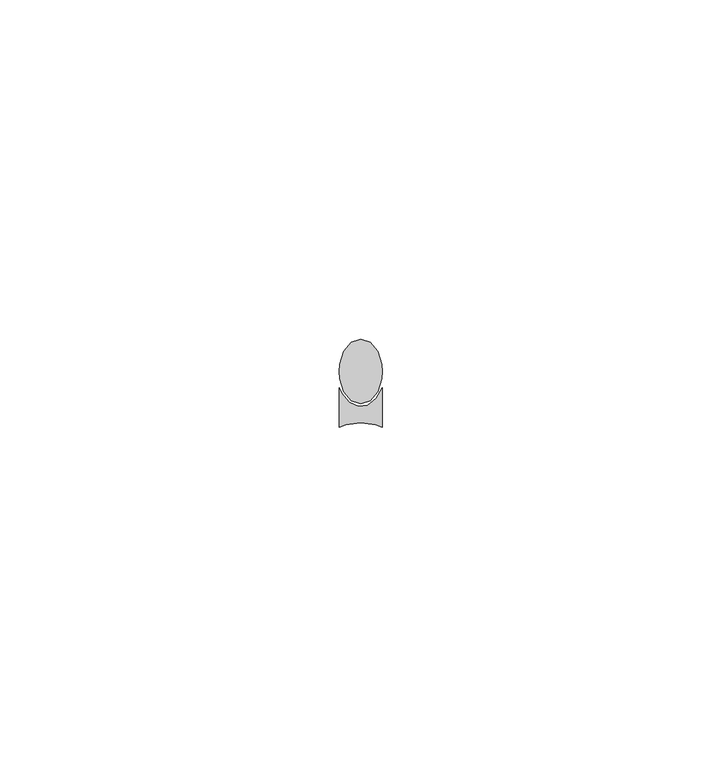
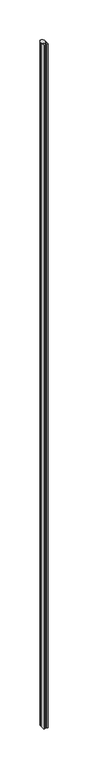
"""IFC4 building model written with IfcOpenShell, lengths in millimetres: proxy geometry, Generic Models 11:Generic Models 1:306267:Generic Models 1:306267 : Generic Models 11:Generic Models 1:306267:300405:Generic Models 1:306267:Generic Models 1:306267 : Generic Models 11:Generic Models 1:306267:300405 : Generic Models 11:Generic Models 1:306267:Generic Models 1:306267 : Generic Models 11:Generic Models 1:306267:300405:21 : Generic Models 11:Generic Models 1:306267:Generic Models 1:306267 : Generic Models 11:Generic Models 1:306267:300405:Generic Models 1:306267:Generic Models 1:306267 : Generic Models 11:Generic Models 1:306267:300405 : Generic Models 11:Generic Models 1:306267:Generic Models 1:306267 : Generic Models 11:Generic Models 1:306267:300405:300182."""

from ifc_helpers import new_model, si_unit, frame, origin, place, context, project, spatial, polyline, outline, extrude, source, transform, mapped, element, save


def generic_models_baf57337(model_context):
    return source(origin(), model_context, "Body", "SweptSolid", [
        extrude(outline(polyline([(593733.5341431, -579092.0005286), (593732.429409, -579090.6790346), (593731.8163278, -579088.7694203), (593731.7367239, -579087.7096644), (593731.8163278, -579086.6499084), (593732.429409, -579084.7402942), (593733.5341431, -579083.4188002), (593734.9117239, -579082.9471644), (593736.2893048, -579083.4188002), (593737.3940389, -579084.7402942), (593738.0071201, -579086.6499084), (593738.0867239, -579087.7096644), (593738.0071201, -579088.7694203), (593737.3940389, -579090.6790346), (593736.2893048, -579092.0005286), (593734.9117239, -579092.4721644), (593733.5341431, -579092.0005286)])), frame((0.0, 0.0, 5106.0759872), z_axis=(0.0, 0.0, 1.0), x_axis=(1.0, 0.0, 0.0)), (0.0, 0.0, 1.0), 1071.4379058),
        extrude(outline(polyline([(593737.1209607, -579095.5639755), (593734.9117239, -579095.2502894), (593732.7024872, -579095.5639755), (593731.7367239, -579095.9413841), (593731.7367239, -579090.073292), (593732.1230415, -579090.9335729), (593733.206527, -579092.2431481), (593734.5567747, -579092.8435016), (593735.962551, -579092.6407137), (593737.2039351, -579091.6665087), (593738.0867239, -579090.073292), (593738.0867239, -579095.9413841), (593737.1209607, -579095.5639755)])), frame((0.0, 0.0, 5106.0759872), z_axis=(0.0, 0.0, 1.0), x_axis=(1.0, 0.0, 0.0)), (0.0, 0.0, 1.0), 1071.4379058),
    ])


if __name__ == "__main__":
    model = new_model("IFC4")
    model_context = context("Model", 3, world=origin())
    ifc_project = project(units=[si_unit("LENGTHUNIT", "METRE", prefix="MILLI")], contexts=[model_context])
    site = spatial("IfcSite", under=ifc_project)
    building = spatial("IfcBuilding", under=site)
    placement = place(None, origin())
    generic_models_shape = generic_models_baf57337(model_context)
    element("IfcBuildingElementProxy", 1, Name="Generic Models 11:Generic Models 1:306267:Generic Models 1:306267 : Generic Models 11:Generic Models 1:306267:300405:Generic Models 1:306267:Generic Models 1:306267 : Generic Models 11:Generic Models 1:306267:300405 : Generic Models 11:Generic Models 1:306267:Generic Models 1:306267 : Generic Models 11:Generic Models 1:306267:300405:21 : Generic Models 11:Generic Models 1:306267:Generic Models 1:306267 : Generic Models 11:Generic Models 1:306267:300405:Generic Models 1:306267:Generic Models 1:306267 : Generic Models 11:Generic Models 1:306267:300405 : Generic Models 11:Generic Models 1:306267:Generic Models 1:306267 : Generic Models 11:Generic Models 1:306267:300405:300182", ObjectType="Generic Models 11:Generic Models 1:306267:Generic Models 1:306267 : Generic Models 11:Generic Models 1:306267:300405:Generic Models 1:306267:Generic Models 1:306267 : Generic Models 11:Generic Models 1:306267:300405 : Generic Models 11:Generic Models 1:306267:Generic Models 1:306267 : Generic Models 11:Generic Models 1:306267:300405:21 : Generic Models 11:Generic Models 1:306267:Generic Models 1:306267 : Generic Models 11:Generic Models 1:306267:300405:Generic Models 1:306267:Generic Models 1:306267 : Generic Models 11:Generic Models 1:306267:300405 : Generic Models 11:Generic Models 1:306267:Generic Models 1:306267 : Generic Models 11:Generic Models 1:306267:300405:300182", at=placement, inside=building, context=model_context, shape_type="MappedRepresentation", body=[
        mapped(generic_models_shape, transform((0.0, 0.0, 0.0), x_axis=(1.0, 0.0, 0.0), y_axis=(0.0, 1.0, 0.0), z_axis=(0.0, 0.0, 1.0))),
    ])
    save(model, "model.ifc")

# Revit data of these elements
# Type "Generic Models 11:Generic Models 1:306267:Generic Models 1:306267 : Generic Models 11:Generic Models 1:306267:300405:Generic Models 1:306267:Generic Models 1:306267 : Generic Models 11:Generic Models 1:306267:300405 : Generic Models 11:Generic Models 1:306267:Generic Models 1:306267 : Generic Models 11:Generic Models 1:306267:300405:21 : Generic Models 11:Generic Models 1:306267:Generic Models 1:306267 : Generic Models 11:Generic Models 1:306267:300405:Generic Models 1:306267:Generic Models 1:306267 : Generic Models 11:Generic Models 1:306267:300405 : Generic Models 11:Generic Models 1:306267:Generic Models 1:306267 : Generic Models 11:Generic Models 1:306267:300405:300182"
#   NameOverride = "Generic Models 11:Generic Models 1:306267:Generic Models 1:306267 : Generic Models 11:Generic Models 1:306267:300405:Generic Models 1:306267:Generic Models 1:306267 : Generic Models 11:Generic Models 1:306267:300405 : Generic Models 11:Generic Models 1:306267:Generic Models 1:306267 : Generic Models 11:Generic Models 1:306267:300405:300182"
#   ObjectTypeOverride = "Generic Models 1:306267:Generic Models 1:306267 : Generic Models 11:Generic Models 1:306267:300405 : Generic Models 11:Generic Models 1:306267:Generic Models 1:306267 : Generic Models 11:Generic Models 1:306267:300405"
#   Reference = "Generic Models 1"
#   Tag = "300182"
# Element 1 (IfcBuildingElementProxy, "Generic Models 11:Generic Models 1:306267:Generic Models 1:306267 : Generic Models 11:Generic Models 1:306267:300405:Generic Models 1:306267:Generic Models 1:306267 : Generic Models 11:Generic Models 1:306267:300405 : Generic Models 11:Generic Models 1:306267:Generic Models 1:306267 : Generic Models 11:Generic Models 1:306267:300405:21 : Generic Models 11:Generic Models 1:306267:Generic Models 1:306267 : Generic Models 11:Generic Models 1:306267:300405:Generic Models 1:306267:Generic Models 1:306267 : Generic Models 11:Generic Models 1:306267:300405 : Generic Models 11:Generic Models 1:306267:Generic Models 1:306267 : Generic Models 11:Generic Models 1:306267:300405:300182")
#   Materials on its faces: "SEALANT & BACKER ROD, IF NECESSARY"
# Materials
#   "SEALANT & BACKER ROD, IF NECESSARY": class "Unassigned", colour RGB 120 120 120, transparency 0, Cost = 0
